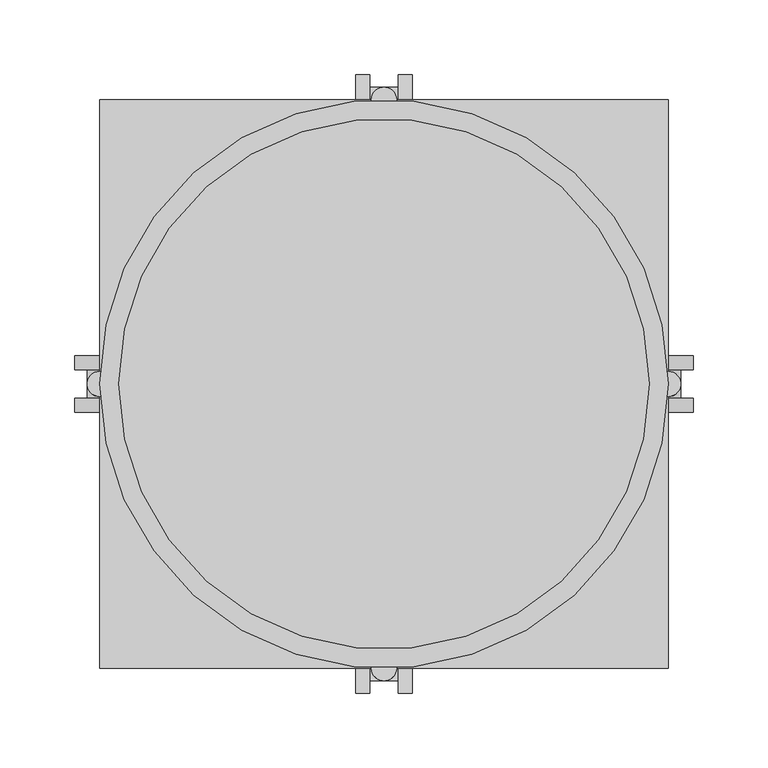
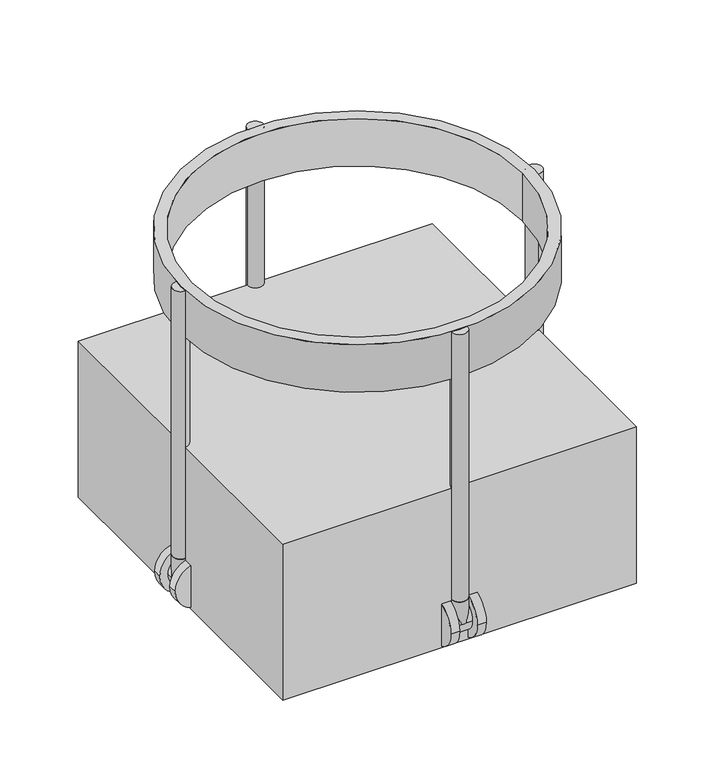
"""IFC4 building model written with IfcOpenShell, lengths in millimetres: proxy geometry, M8900 - Carriage, Pail, CRS, Without Pail : M8900 - Carriage, Pail, CRS, Without Pail."""

import ifcopenshell
import ifcopenshell.guid

model = None  # the IFC model being written
_history = None  # IfcOwnerHistory: only IFC2X3 demands one
_inside = {}  # id of a spatial element -> (the spatial element, [elements in it])
_under = {}  # id of a project, library or spatial element -> (it, [spatial elements below it])
_declared = {}  # id of a project -> (the project, [libraries it declares])
_typed = {}  # id of a type object -> (the type object, [elements of that type])
_made_of = {}  # id of a material, layer set ... -> (it, [elements and type objects made of it])


def new_model(schema):
    """Start an empty IFC model of exactly this schema.

    Asked for "IFC4X3", IfcOpenShell would pick the latest addendum, in which some entities
    have other attributes; the version numbers below select the first issue.
    IFC2X3 requires an IfcOwnerHistory on every rooted entity: one is made here for all.
    """
    global model, _history
    if schema == "IFC4X3":
        model = ifcopenshell.file(schema_version=(4, 3, 0, 0))
    else:
        model = ifcopenshell.file(schema=schema)
    _inside.clear()
    _under.clear()
    _declared.clear()
    _typed.clear()
    _made_of.clear()
    _history = None
    if model.schema == "IFC2X3":
        org = make("IfcOrganization", Name="unknown")
        user = make(
            "IfcPersonAndOrganization",
            ThePerson=make("IfcPerson", FamilyName="unknown"),
            TheOrganization=org,
        )
        app = make(
            "IfcApplication",
            ApplicationDeveloper=org,
            Version="unknown",
            ApplicationFullName="unknown",
            ApplicationIdentifier="unknown",
        )
        _history = make(
            "IfcOwnerHistory",
            OwningUser=user,
            OwningApplication=app,
            ChangeAction="ADDED",
            CreationDate=0,
        )
    return model


def make(cls, **values):
    """One entity of the class cls with the attributes given. An attribute that is None is left unset."""
    return model.create_entity(
        cls, **{name: value for name, value in values.items() if value is not None}
    )


def rooted(cls, **values):
    """An entity with a GlobalId (a new one), such as an element, a storey or a relation."""
    return make(cls, GlobalId=ifcopenshell.guid.new(), OwnerHistory=_history, **values)


def si_unit(unit_type, name, prefix=None):
    """IfcSIUnit, for example si_unit("LENGTHUNIT", "METRE", prefix="MILLI")."""
    return make("IfcSIUnit", UnitType=unit_type, Prefix=prefix, Name=name)


def assignment(units):
    """IfcUnitAssignment: the units of a project."""
    return None if units is None else make("IfcUnitAssignment", Units=units)


def point(xyz):
    """IfcCartesianPoint."""
    return None if xyz is None else make("IfcCartesianPoint", Coordinates=xyz)


def direction(xyz):
    """IfcDirection."""
    return None if xyz is None else make("IfcDirection", DirectionRatios=xyz)


def frame(location, z_axis=None, x_axis=None):
    """IfcAxis2Placement3D, a coordinate frame: its origin and axes. An axis left out is left unset."""
    return make(
        "IfcAxis2Placement3D",
        Location=point(location),
        Axis=direction(z_axis),
        RefDirection=direction(x_axis),
    )


def frame_2d(location, x_axis=None):
    """IfcAxis2Placement2D, a coordinate frame in the plane: its origin and x axis."""
    return make(
        "IfcAxis2Placement2D", Location=point(location), RefDirection=direction(x_axis)
    )


def origin():
    """The frame at (0, 0, 0) with its axes left unset."""
    return frame((0.0, 0.0, 0.0))


def origin_with_axes():
    """The frame at (0, 0, 0) with the z axis (0, 0, 1) and the x axis (1, 0, 0) written out."""
    return frame((0.0, 0.0, 0.0), z_axis=(0.0, 0.0, 1.0), x_axis=(1.0, 0.0, 0.0))


def origin_2d():
    """The frame at (0, 0) in the plane with its x axis left unset."""
    return frame_2d((0.0, 0.0))


def place(relative_to, where):
    """IfcLocalPlacement: puts the frame where relative to a parent placement (None: the world)."""
    return make(
        "IfcLocalPlacement", PlacementRelTo=relative_to, RelativePlacement=where
    )


def context(
    kind, dimensions, precision=None, world=None, true_north=None, identifier=None
):
    """IfcGeometricRepresentationContext, for example the 3D "Model" context."""
    return make(
        "IfcGeometricRepresentationContext",
        ContextIdentifier=identifier,
        ContextType=kind,
        CoordinateSpaceDimension=dimensions,
        Precision=precision,
        WorldCoordinateSystem=world,
        TrueNorth=true_north,
    )


def project(units=None, contexts=None):
    """IfcProject with its units and contexts."""
    return rooted(
        "IfcProject",
        Name="project",
        RepresentationContexts=contexts,
        UnitsInContext=assignment(units),
    )


def spatial(cls, under=None, at=None, **own):
    """A site, building, storey or space (cls), placed at a placement, below another one or the project."""
    s = rooted(cls, ObjectPlacement=at, **own)
    if under is not None:
        _under.setdefault(under.id(), (under, []))[1].append(s)
    return s


def polyline(points):
    """IfcPolyline through the points."""
    return make("IfcPolyline", Points=[point(p) for p in points])


def circle_curve(where, radius):
    """IfcCircle in the frame where."""
    return make("IfcCircle", Position=where, Radius=radius)


def trimmed(basis, trim1, trim2, sense, master):
    """IfcTrimmedCurve: the piece of a basis curve between two trims."""
    return make(
        "IfcTrimmedCurve",
        BasisCurve=basis,
        Trim1=trim1,
        Trim2=trim2,
        SenseAgreement=sense,
        MasterRepresentation=master,
    )


def segment(curve, same_sense, transition):
    """IfcCompositeCurveSegment."""
    return make(
        "IfcCompositeCurveSegment",
        Transition=transition,
        SameSense=same_sense,
        ParentCurve=curve,
    )


def composite_curve(segments, self_intersect=None):
    """IfcCompositeCurve: segments joined end to end."""
    return make("IfcCompositeCurve", Segments=segments, SelfIntersect=self_intersect)


def outline(outer, holes=None, kind="AREA"):
    """IfcArbitraryClosedProfileDef: a profile drawn as a closed curve; with holes, ...WithVoids."""
    if holes is None:
        return make("IfcArbitraryClosedProfileDef", ProfileType=kind, OuterCurve=outer)
    return make(
        "IfcArbitraryProfileDefWithVoids",
        ProfileType=kind,
        OuterCurve=outer,
        InnerCurves=holes,
    )


def extrude(swept, where, along, depth):
    """IfcExtrudedAreaSolid: the profile swept, set in the frame where, extruded along a direction by depth."""
    return make(
        "IfcExtrudedAreaSolid",
        SweptArea=swept,
        Position=where,
        ExtrudedDirection=direction(along),
        Depth=depth,
    )


def shape(context_of_items, identifier, shape_type, items):
    """IfcShapeRepresentation: the items that make up one representation, for example the "Body"."""
    return make(
        "IfcShapeRepresentation",
        ContextOfItems=context_of_items,
        RepresentationIdentifier=identifier,
        RepresentationType=shape_type,
        Items=items,
    )


def source(mapping_origin, context_of_items, identifier, shape_type, items):
    """IfcRepresentationMap: a shape defined once, which mapped items show again and again."""
    return make(
        "IfcRepresentationMap",
        MappingOrigin=mapping_origin,
        MappedRepresentation=shape(context_of_items, identifier, shape_type, items),
    )


def transform(
    local_origin,
    x_axis=None,
    y_axis=None,
    z_axis=None,
    scale=None,
    scale2=None,
    scale3=None,
    uniform=True,
):
    """IfcCartesianTransformationOperator3D, or its non-uniform kind. x_axis, y_axis, z_axis: its Axis1, 2, 3."""
    if uniform:
        return make(
            "IfcCartesianTransformationOperator3D",
            Axis1=direction(x_axis),
            Axis2=direction(y_axis),
            LocalOrigin=point(local_origin),
            Scale=scale,
            Axis3=direction(z_axis),
        )
    return make(
        "IfcCartesianTransformationOperator3DnonUniform",
        Axis1=direction(x_axis),
        Axis2=direction(y_axis),
        LocalOrigin=point(local_origin),
        Scale=scale,
        Axis3=direction(z_axis),
        Scale2=scale2,
        Scale3=scale3,
    )


def mapped(mapping_source, mapping_target):
    """IfcMappedItem: shows the shape of a source again, moved by a transform."""
    return make(
        "IfcMappedItem", MappingSource=mapping_source, MappingTarget=mapping_target
    )


def made_of(thing, what):
    """Note that an element or type object is made of a material, layer set ...; save() writes the relation."""
    if what is not None:
        _made_of.setdefault(what.id(), (what, []))[1].append(thing)
    return thing


def element(
    cls,
    number,
    at=None,
    inside=None,
    cuts=None,
    type_object=None,
    material=None,
    context=None,
    identifier="Body",
    shape_type=None,
    held_by="IfcProductDefinitionShape",
    body=None,
    shapes=None,
    **own,
):
    """One element of the class cls, such as IfcWall. Its Tag is "e" and its number.

    at: its placement. inside: the storey or other place that contains it. cuts: it is an
    opening in that element (IfcRelVoidsElement). A single representation is given by context,
    identifier, shape_type and body (its items); several are given by shapes. held_by: the class
    of the entity that holds the representations. save() writes the other relations.
    """
    e = rooted(cls, Tag="e%d" % number, ObjectPlacement=at, **own)
    if body is not None:
        shapes = [shape(context, identifier, shape_type, body)]
    if shapes is not None:
        e.Representation = make(held_by, Representations=shapes)
    if inside is not None:
        _inside.setdefault(inside.id(), (inside, []))[1].append(e)
    if cuts is not None:
        rooted(
            "IfcRelVoidsElement", RelatingBuildingElement=cuts, RelatedOpeningElement=e
        )
    if type_object is not None:
        _typed.setdefault(type_object.id(), (type_object, []))[1].append(e)
    return made_of(e, material)


def aggregate(whole, parts):
    """IfcRelAggregates: a whole, such as a stair, and the parts it consists of."""
    return rooted("IfcRelAggregates", RelatingObject=whole, RelatedObjects=parts)


def save(model, path):
    """Write the relations noted so far, then the file.

    IfcRelAggregates (storeys below a building ...), IfcRelContainedInSpatialStructure (elements
    in a storey), IfcRelDefinesByType, IfcRelAssociatesMaterial and IfcRelDeclares: one each for
    every whole, place, type object, material and project.
    """
    for whole, parts in _under.values():
        aggregate(whole, parts)
    for where, things in _inside.values():
        rooted(
            "IfcRelContainedInSpatialStructure",
            RelatedElements=things,
            RelatingStructure=where,
        )
    for kind, things in _typed.values():
        rooted("IfcRelDefinesByType", RelatedObjects=things, RelatingType=kind)
    for what, things in _made_of.values():
        rooted("IfcRelAssociatesMaterial", RelatedObjects=things, RelatingMaterial=what)
    for by, libraries in _declared.values():
        rooted("IfcRelDeclares", RelatingContext=by, RelatedDefinitions=libraries)
    model.write(path)


def specialty_equipment_7e218527(model_context):
    return source(origin(), model_context, "Body", "SweptSolid", [
        extrude(outline(composite_curve([segment(trimmed(circle_curve(origin_2d(), 190.5), [point((-190.5, 0.0))], [point((190.5, 0.0))], False, "CARTESIAN"), True, "CONTINUOUS"), segment(trimmed(circle_curve(origin_2d(), 190.5), [point((190.5, 0.0))], [point((-190.5, 0.0))], False, "CARTESIAN"), True, "CONTINUOUS")], self_intersect=False), holes=[composite_curve([segment(trimmed(circle_curve(origin_2d(), 177.8), [point((-177.8, 0.0))], [point((177.8, 0.0))], True, "CARTESIAN"), True, "CONTINUOUS"), segment(trimmed(circle_curve(origin_2d(), 177.8), [point((177.8, 0.0))], [point((-177.8, 0.0))], True, "CARTESIAN"), True, "CONTINUOUS")], self_intersect=False)]), frame((0.0, 0.0, 301.694085), z_axis=(0.0, 0.0, 1.0), x_axis=(1.0, 0.0, 0.0)), (0.0, 0.0, 1.0), 53.905915),
        extrude(outline(composite_curve([segment(trimmed(circle_curve(frame_2d((25.4, -182.0333333)), 25.4), [point((25.4, -156.6333333))], [point((25.4, -207.4333333))], False, "CARTESIAN"), True, "CONTINUOUS"), segment(trimmed(circle_curve(frame_2d((25.4, -182.0333333)), 25.4), [point((25.4, -207.4333333))], [point((25.4, -156.6333333))], False, "CARTESIAN"), True, "CONTINUOUS")], self_intersect=False)), frame((0.0, -19.05, 0.0), z_axis=(0.0, 1.0, 0.0), x_axis=(0.0, 0.0, 1.0)), (0.0, 0.0, 1.0), 9.525),
        extrude(outline(composite_curve([segment(trimmed(circle_curve(frame_2d((25.4, -182.0333333)), 25.4), [point((25.4, -156.6333333))], [point((25.4, -207.4333333))], False, "CARTESIAN"), True, "CONTINUOUS"), segment(trimmed(circle_curve(frame_2d((25.4, -182.0333333)), 25.4), [point((25.4, -207.4333333))], [point((25.4, -156.6333333))], False, "CARTESIAN"), True, "CONTINUOUS")], self_intersect=False)), frame((0.0, 9.525, 0.0), z_axis=(0.0, 1.0, 0.0), x_axis=(0.0, 0.0, 1.0)), (0.0, 0.0, 1.0), 9.525),
        extrude(outline(composite_curve([segment(trimmed(circle_curve(frame_2d((-190.5, 0.0)), 8.4666667), [point((-190.5, 8.4666667))], [point((-190.5, -8.4666667))], False, "CARTESIAN"), True, "CONTINUOUS"), segment(trimmed(circle_curve(frame_2d((-190.5, 0.0)), 8.4666667), [point((-190.5, -8.4666667))], [point((-190.5, 8.4666667))], False, "CARTESIAN"), True, "CONTINUOUS")], self_intersect=False)), frame((0.0, 0.0, 25.4), z_axis=(0.0, 0.0, 1.0), x_axis=(1.0, 0.0, 0.0)), (0.0, 0.0, 1.0), 25.4),
        extrude(outline(composite_curve([segment(trimmed(circle_curve(frame_2d((25.4, -182.0333333)), 16.9333333), [point((25.4, -165.1))], [point((25.4, -198.9666667))], False, "CARTESIAN"), True, "CONTINUOUS"), segment(trimmed(circle_curve(frame_2d((25.4, -182.0333333)), 16.9333333), [point((25.4, -198.9666667))], [point((25.4, -165.1))], False, "CARTESIAN"), True, "CONTINUOUS")], self_intersect=False)), frame((0.0, -9.525, 0.0), z_axis=(0.0, 1.0, 0.0), x_axis=(0.0, 0.0, 1.0)), (0.0, 0.0, 1.0), 19.05),
        extrude(outline(composite_curve([segment(trimmed(circle_curve(frame_2d((25.4, 182.0333333)), 25.4), [point((25.4, 156.6333333))], [point((25.4, 207.4333333))], False, "CARTESIAN"), True, "CONTINUOUS"), segment(trimmed(circle_curve(frame_2d((25.4, 182.0333333)), 25.4), [point((25.4, 207.4333333))], [point((25.4, 156.6333333))], False, "CARTESIAN"), True, "CONTINUOUS")], self_intersect=False)), frame((0.0, -19.05, 0.0), z_axis=(0.0, 1.0, 0.0), x_axis=(0.0, 0.0, 1.0)), (0.0, 0.0, 1.0), 9.525),
        extrude(outline(composite_curve([segment(trimmed(circle_curve(frame_2d((25.4, 182.0333333)), 25.4), [point((25.4, 156.6333333))], [point((25.4, 207.4333333))], False, "CARTESIAN"), True, "CONTINUOUS"), segment(trimmed(circle_curve(frame_2d((25.4, 182.0333333)), 25.4), [point((25.4, 207.4333333))], [point((25.4, 156.6333333))], False, "CARTESIAN"), True, "CONTINUOUS")], self_intersect=False)), frame((0.0, 9.525, 0.0), z_axis=(0.0, 1.0, 0.0), x_axis=(0.0, 0.0, 1.0)), (0.0, 0.0, 1.0), 9.525),
        extrude(outline(composite_curve([segment(trimmed(circle_curve(frame_2d((190.5, 0.0)), 8.4666667), [point((190.5, 8.4666667))], [point((190.5, -8.4666667))], False, "CARTESIAN"), True, "CONTINUOUS"), segment(trimmed(circle_curve(frame_2d((190.5, 0.0)), 8.4666667), [point((190.5, -8.4666667))], [point((190.5, 8.4666667))], False, "CARTESIAN"), True, "CONTINUOUS")], self_intersect=False)), frame((0.0, 0.0, 25.4), z_axis=(0.0, 0.0, 1.0), x_axis=(1.0, 0.0, 0.0)), (0.0, 0.0, 1.0), 25.4),
        extrude(outline(composite_curve([segment(trimmed(circle_curve(frame_2d((25.4, 182.0333333)), 16.9333333), [point((25.4, 165.1))], [point((25.4, 198.9666667))], False, "CARTESIAN"), True, "CONTINUOUS"), segment(trimmed(circle_curve(frame_2d((25.4, 182.0333333)), 16.9333333), [point((25.4, 198.9666667))], [point((25.4, 165.1))], False, "CARTESIAN"), True, "CONTINUOUS")], self_intersect=False)), frame((0.0, -9.525, 0.0), z_axis=(0.0, 1.0, 0.0), x_axis=(0.0, 0.0, 1.0)), (0.0, 0.0, 1.0), 19.05),
        extrude(outline(composite_curve([segment(trimmed(circle_curve(frame_2d((-182.0333333, 25.4)), 25.4), [point((-156.6333333, 25.4))], [point((-207.4333333, 25.4))], False, "CARTESIAN"), True, "CONTINUOUS"), segment(trimmed(circle_curve(frame_2d((-182.0333333, 25.4)), 25.4), [point((-207.4333333, 25.4))], [point((-156.6333333, 25.4))], False, "CARTESIAN"), True, "CONTINUOUS")], self_intersect=False)), frame((9.525, 0.0, 0.0), z_axis=(1.0, 0.0, 0.0), x_axis=(0.0, 1.0, 0.0)), (0.0, 0.0, 1.0), 9.525),
        extrude(outline(composite_curve([segment(trimmed(circle_curve(frame_2d((-182.0333333, 25.4)), 25.4), [point((-156.6333333, 25.4))], [point((-207.4333333, 25.4))], False, "CARTESIAN"), True, "CONTINUOUS"), segment(trimmed(circle_curve(frame_2d((-182.0333333, 25.4)), 25.4), [point((-207.4333333, 25.4))], [point((-156.6333333, 25.4))], False, "CARTESIAN"), True, "CONTINUOUS")], self_intersect=False)), frame((-19.05, 0.0, 0.0), z_axis=(1.0, 0.0, 0.0), x_axis=(0.0, 1.0, 0.0)), (0.0, 0.0, 1.0), 9.525),
        extrude(outline(composite_curve([segment(trimmed(circle_curve(frame_2d((0.0, -190.5)), 8.4666667), [point((-8.4666667, -190.5))], [point((8.4666667, -190.5))], False, "CARTESIAN"), True, "CONTINUOUS"), segment(trimmed(circle_curve(frame_2d((0.0, -190.5)), 8.4666667), [point((8.4666667, -190.5))], [point((-8.4666667, -190.5))], False, "CARTESIAN"), True, "CONTINUOUS")], self_intersect=False)), frame((0.0, 0.0, 25.4), z_axis=(0.0, 0.0, 1.0), x_axis=(1.0, 0.0, 0.0)), (0.0, 0.0, 1.0), 25.4),
        extrude(outline(composite_curve([segment(trimmed(circle_curve(frame_2d((-182.0333333, 25.4)), 16.9333333), [point((-165.1, 25.4))], [point((-198.9666667, 25.4))], False, "CARTESIAN"), True, "CONTINUOUS"), segment(trimmed(circle_curve(frame_2d((-182.0333333, 25.4)), 16.9333333), [point((-198.9666667, 25.4))], [point((-165.1, 25.4))], False, "CARTESIAN"), True, "CONTINUOUS")], self_intersect=False)), frame((-9.525, 0.0, 0.0), z_axis=(1.0, 0.0, 0.0), x_axis=(0.0, 1.0, 0.0)), (0.0, 0.0, 1.0), 19.05),
        extrude(outline(composite_curve([segment(trimmed(circle_curve(frame_2d((182.0333333, 25.4)), 25.4), [point((156.6333333, 25.4))], [point((207.4333333, 25.4))], False, "CARTESIAN"), True, "CONTINUOUS"), segment(trimmed(circle_curve(frame_2d((182.0333333, 25.4)), 25.4), [point((207.4333333, 25.4))], [point((156.6333333, 25.4))], False, "CARTESIAN"), True, "CONTINUOUS")], self_intersect=False)), frame((9.525, 0.0, 0.0), z_axis=(1.0, 0.0, 0.0), x_axis=(0.0, 1.0, 0.0)), (0.0, 0.0, 1.0), 9.525),
        extrude(outline(composite_curve([segment(trimmed(circle_curve(frame_2d((182.0333333, 25.4)), 25.4), [point((156.6333333, 25.4))], [point((207.4333333, 25.4))], False, "CARTESIAN"), True, "CONTINUOUS"), segment(trimmed(circle_curve(frame_2d((182.0333333, 25.4)), 25.4), [point((207.4333333, 25.4))], [point((156.6333333, 25.4))], False, "CARTESIAN"), True, "CONTINUOUS")], self_intersect=False)), frame((-19.05, 0.0, 0.0), z_axis=(1.0, 0.0, 0.0), x_axis=(0.0, 1.0, 0.0)), (0.0, 0.0, 1.0), 9.525),
        extrude(outline(composite_curve([segment(trimmed(circle_curve(frame_2d((0.0, 190.5)), 8.4666667), [point((-8.4666667, 190.5))], [point((8.4666667, 190.5))], False, "CARTESIAN"), True, "CONTINUOUS"), segment(trimmed(circle_curve(frame_2d((0.0, 190.5)), 8.4666667), [point((8.4666667, 190.5))], [point((-8.4666667, 190.5))], False, "CARTESIAN"), True, "CONTINUOUS")], self_intersect=False)), frame((0.0, 0.0, 25.4), z_axis=(0.0, 0.0, 1.0), x_axis=(1.0, 0.0, 0.0)), (0.0, 0.0, 1.0), 25.4),
        extrude(outline(composite_curve([segment(trimmed(circle_curve(frame_2d((182.0333333, 25.4)), 16.9333333), [point((165.1, 25.4))], [point((198.9666667, 25.4))], False, "CARTESIAN"), True, "CONTINUOUS"), segment(trimmed(circle_curve(frame_2d((182.0333333, 25.4)), 16.9333333), [point((198.9666667, 25.4))], [point((165.1, 25.4))], False, "CARTESIAN"), True, "CONTINUOUS")], self_intersect=False)), frame((-9.525, 0.0, 0.0), z_axis=(1.0, 0.0, 0.0), x_axis=(0.0, 1.0, 0.0)), (0.0, 0.0, 1.0), 19.05),
        extrude(outline(composite_curve([segment(trimmed(circle_curve(frame_2d((-190.5, 0.0)), 8.4666667), [point((-190.5, 8.4666667))], [point((-190.5, -8.4666667))], False, "CARTESIAN"), True, "CONTINUOUS"), segment(trimmed(circle_curve(frame_2d((-190.5, 0.0)), 8.4666667), [point((-190.5, -8.4666667))], [point((-190.5, 8.4666667))], False, "CARTESIAN"), True, "CONTINUOUS")], self_intersect=False)), frame((0.0, 0.0, 50.8), z_axis=(0.0, 0.0, 1.0), x_axis=(1.0, 0.0, 0.0)), (0.0, 0.0, 1.0), 304.8),
        extrude(outline(composite_curve([segment(trimmed(circle_curve(frame_2d((0.0, 190.5)), 8.4666667), [point((8.4666667, 190.5))], [point((-8.4666667, 190.5))], False, "CARTESIAN"), True, "CONTINUOUS"), segment(trimmed(circle_curve(frame_2d((0.0, 190.5)), 8.4666667), [point((-8.4666667, 190.5))], [point((8.4666667, 190.5))], False, "CARTESIAN"), True, "CONTINUOUS")], self_intersect=False)), frame((0.0, 0.0, 50.8), z_axis=(0.0, 0.0, 1.0), x_axis=(1.0, 0.0, 0.0)), (0.0, 0.0, 1.0), 304.8),
        extrude(outline(composite_curve([segment(trimmed(circle_curve(frame_2d((190.5, 0.0)), 8.4666667), [point((190.5, -8.4666667))], [point((190.5, 8.4666667))], False, "CARTESIAN"), True, "CONTINUOUS"), segment(trimmed(circle_curve(frame_2d((190.5, 0.0)), 8.4666667), [point((190.5, 8.4666667))], [point((190.5, -8.4666667))], False, "CARTESIAN"), True, "CONTINUOUS")], self_intersect=False)), frame((0.0, 0.0, 50.8), z_axis=(0.0, 0.0, 1.0), x_axis=(1.0, 0.0, 0.0)), (0.0, 0.0, 1.0), 304.8),
        extrude(outline(composite_curve([segment(trimmed(circle_curve(frame_2d((0.0, -190.5)), 8.4666667), [point((-8.4666667, -190.5))], [point((8.4666667, -190.5))], False, "CARTESIAN"), True, "CONTINUOUS"), segment(trimmed(circle_curve(frame_2d((0.0, -190.5)), 8.4666667), [point((8.4666667, -190.5))], [point((-8.4666667, -190.5))], False, "CARTESIAN"), True, "CONTINUOUS")], self_intersect=False)), frame((0.0, 0.0, 50.8), z_axis=(0.0, 0.0, 1.0), x_axis=(1.0, 0.0, 0.0)), (0.0, 0.0, 1.0), 304.8),
        extrude(outline(polyline([(-190.5, 190.5), (190.5, 190.5), (190.5, -190.5), (-190.5, -190.5), (-190.5, 0.0), (-190.5, 190.5)])), origin_with_axes(), (0.0, 0.0, 1.0), 177.8),
    ])


if __name__ == "__main__":
    model = new_model("IFC4")
    model_context = context("Model", 3, world=origin())
    ifc_project = project(units=[si_unit("LENGTHUNIT", "METRE", prefix="MILLI")], contexts=[model_context])
    site = spatial("IfcSite", under=ifc_project)
    building = spatial("IfcBuilding", under=site)
    placement = place(None, origin())
    specialty_equipment_shape = specialty_equipment_7e218527(model_context)
    element("IfcBuildingElementProxy", 1, Name="M8900 - Carriage, Pail, CRS, Without Pail : M8900 - Carriage, Pail, CRS, Without Pail", ObjectType="M8900 - Carriage, Pail, CRS, Without Pail : M8900 - Carriage, Pail, CRS, Without Pail", at=placement, inside=building, context=model_context, shape_type="MappedRepresentation", body=[
        mapped(specialty_equipment_shape, transform((0.0, 0.0, 0.0), x_axis=(1.0, 0.0, 0.0), y_axis=(0.0, 1.0, 0.0), z_axis=(0.0, 0.0, 1.0))),
    ])
    save(model, "model.ifc")

# Revit data of these elements
# Type "M8900 - Carriage, Pail, CRS, Without Pail : M8900 - Carriage, Pail, CRS, Without Pail"
#   Watts2 = "0"
#   Watts1 = "0"
#   Unit_Issue = "EA"
#   UTIL_6_Misc = "-"
#   UTIL_5_NonMedGas = "-"
#   UTIL_4_MiscGas = "-"
#   UTIL_3_MedGas = "-"
#   UTIL_2_Elec = "-"
#   UTIL_1_WaterDrain = "-"
#   Nomenclature = "Carriage, Pail, CRS, Without Pail"
#   NSN = "6530"
#   Location [instance default] = ""
#   JSN = "M8900"
#   Fund_Source_VA = "-"
#   Fund_Source_Navy = "-"
#   Fund_Source_Army = "-"
#   Fund_Source_AF = "-"
#   ELEC_Volts2 = "0"
#   ELEC_Volts1 = "0"
#   ELEC_Phase2 = "0"
#   ELEC_Phase1 = "0"
#   ELEC_HertzSwitch = "0"
#   ELEC_HertzDependent = "0"
#   ELEC_Hertz = "0"
#   ELEC_Amps2 = "0"
#   ELEC_Amps1 = "0"
#   DetailDescription = "Carriage, pail (kick bucket) CRS. Consists of a stainless steel ring type carriage mounted on ball bearing casters. Includes circular nonmarring bumper. For use in the surgical operating room."
#   CAT_VA = "C"
#   CAT_Navy = "C"
#   CAT_IHS = "-"
#   CAT_Army = "C"
#   CAT_AF = "C"
#   BTUperhour = "0"
#   radius2 = 0' - 7"
#   radius = 0' - 7 1/2"
#   calc 2 = 0' - 0.33333"
#   calc 1 = 0' - 0.66667"
#   Weight_IP = 8
#   DIM_Width_IP = 1' - 3"
#   DIM_Height_IP = 0' - 7"
#   DIM_Depth_IP = 1' - 3"
#   finish [instance default] = none
# Element 1 (IfcBuildingElementProxy, "M8900 - Carriage, Pail, CRS, Without Pail : M8900 - Carriage, Pail, CRS, Without Pail")
#   Location = "TRPE1"
#   Materials on its faces: "EquipSpace"
# Materials
#   "EquipSpace": class "Unassigned", colour RGB 221 217 195, transparency 0.5
